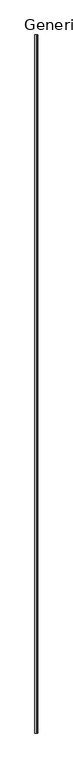
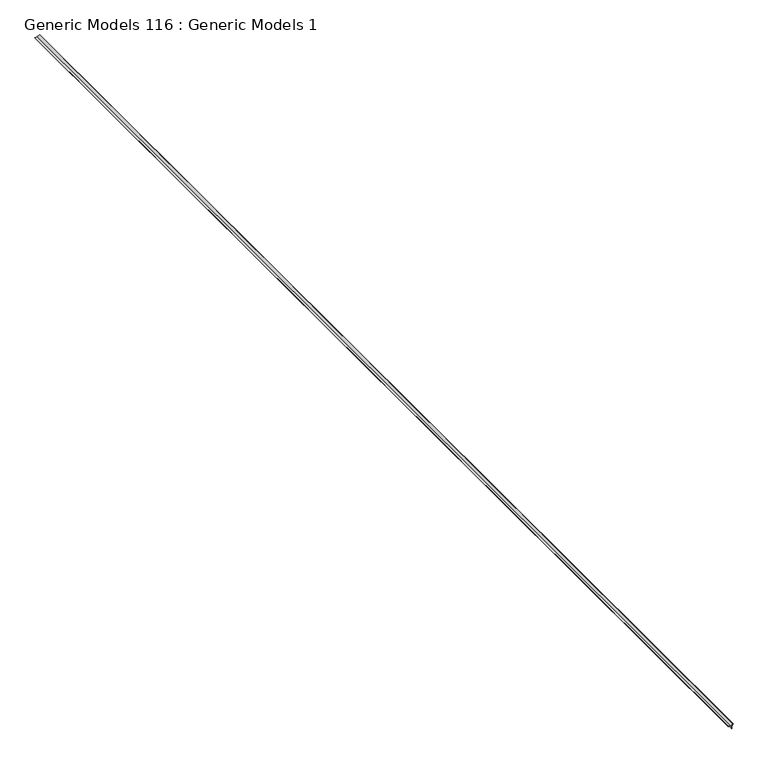
"""IFC4 building model written with IfcOpenShell, lengths in millimetres: proxy geometry, Generic Models 116 : Generic Models 1."""

from ifc_helpers import new_model, si_unit, point, frame, frame_2d, origin, place, context, project, spatial, polyline, circle_curve, trimmed, segment, composite_curve, outline, extrude, source, transform, mapped, element, save


def generic_models_116_generic_models_1_d4966e75(model_context):
    return source(origin(), model_context, "Body", "SweptSolid", [
        extrude(outline(composite_curve([segment(polyline([(127128.4926156, 7314.9518851), (127108.966, 7276.9263704), (127108.966, 7238.8263704), (127107.696, 7238.8263704), (127107.696, 7277.2333942), (127127.5962396, 7315.9864925), (127088.8431414, 7296.0862528), (127050.4361176, 7296.0862528), (127050.4361176, 7297.3562528), (127088.5361176, 7297.3562528), (127126.5616323, 7316.8828684)]), True, "CONTINUOUS"), segment(trimmed(circle_curve(frame_2d((127127.2167873, 7315.6070401)), 1.4342127), [point((127126.5616323, 7316.8828684))], [point((127128.4926156, 7314.9518851))], False, "CARTESIAN"), True, "CONTINUOUS")], self_intersect=False)), frame((0.0, -7068.1230338, 0.0), z_axis=(0.0, 1.0, 0.0), x_axis=(0.0, 0.0, 1.0)), (0.0, 0.0, 1.0), 19050.0),
    ])


if __name__ == "__main__":
    model = new_model("IFC4")
    model_context = context("Model", 3, world=origin())
    ifc_project = project(units=[si_unit("LENGTHUNIT", "METRE", prefix="MILLI")], contexts=[model_context])
    site = spatial("IfcSite", under=ifc_project)
    building = spatial("IfcBuilding", under=site)
    placement = place(None, origin())
    generic_models_116_generic_models_1_shape = generic_models_116_generic_models_1_d4966e75(model_context)
    element("IfcBuildingElementProxy", 1, Name="Generic Models 116 : Generic Models 1", ObjectType="Generic Models 116 : Generic Models 1", at=placement, inside=building, context=model_context, shape_type="MappedRepresentation", body=[
        mapped(generic_models_116_generic_models_1_shape, transform((0.0, 0.0, 0.0), x_axis=(1.0, 0.0, 0.0), y_axis=(0.0, 1.0, 0.0), z_axis=(0.0, 0.0, 1.0))),
    ])
    save(model, "model.ifc")

# Revit data of these elements
# Element 1 (IfcBuildingElementProxy, "Generic Models 116 : Generic Models 1")
#   Materials on its faces: "_CONTINUOUS 16 GA. COPPER CORNER BEAD"
# Materials
#   "_CONTINUOUS 16 GA. COPPER CORNER BEAD": class "Generic", colour RGB 253 192 103, transparency 0, Cost = 0
